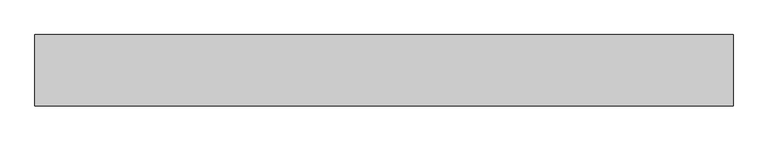
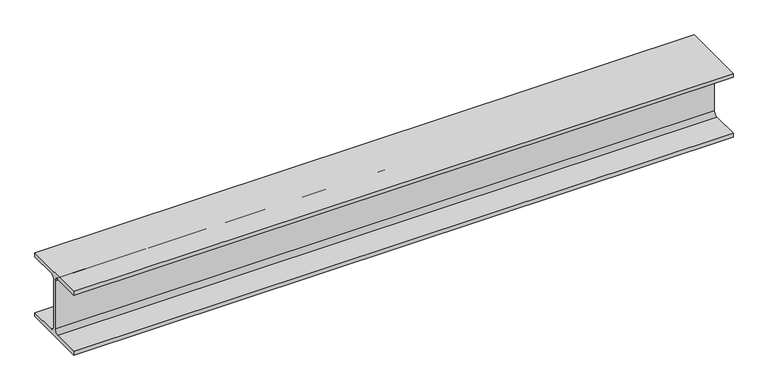
"""IFC4 building model written with IfcOpenShell, lengths in millimetres: beam geometry, 0912_Steel Framing_H-KSD3502 : H_SB_ASB_H-200x200x8x12."""

from ifc_helpers import new_model, si_unit, point, frame, frame_2d, origin, place, context, project, spatial, polyline, circle_curve, trimmed, segment, composite_curve, outline, extrude, source, transform, mapped, element, save


def beam_1032c180(model_context):
    return source(origin(), model_context, "Body", "SweptSolid", [
        extrude(outline(composite_curve([segment(polyline([(100.0, -88.0), (100.0, -100.0), (-100.0, -100.0), (-100.0, -88.0), (-17.0, -88.0)]), True, "CONTINUOUS"), segment(trimmed(circle_curve(frame_2d((-17.0, -75.0)), 13.0), [point((-17.0, -88.0))], [point((-4.0, -75.0))], True, "CARTESIAN"), True, "CONTINUOUS"), segment(polyline([(-4.0, -75.0), (-4.0, 75.0)]), True, "CONTINUOUS"), segment(trimmed(circle_curve(frame_2d((-17.0, 75.0)), 13.0), [point((-4.0, 75.0))], [point((-17.0, 88.0))], True, "CARTESIAN"), True, "CONTINUOUS"), segment(polyline([(-17.0, 88.0), (-100.0, 88.0), (-100.0, 100.0), (100.0, 100.0), (100.0, 88.0), (17.0, 88.0)]), True, "CONTINUOUS"), segment(trimmed(circle_curve(frame_2d((17.0, 75.0)), 13.0), [point((17.0, 88.0))], [point((4.0, 75.0))], True, "CARTESIAN"), True, "CONTINUOUS"), segment(polyline([(4.0, 75.0), (4.0, -75.0)]), True, "CONTINUOUS"), segment(trimmed(circle_curve(frame_2d((17.0, -75.0)), 13.0), [point((4.0, -75.0))], [point((17.0, -88.0))], True, "CARTESIAN"), True, "CONTINUOUS"), segment(polyline([(17.0, -88.0), (100.0, -88.0)]), True, "CONTINUOUS")], self_intersect=False)), frame((-926.5182437, 0.0, 0.0), z_axis=(1.0, 0.0, 0.0), x_axis=(0.0, 1.0, 0.0)), (0.0, 0.0, 1.0), 1959.1715213),
    ])


if __name__ == "__main__":
    model = new_model("IFC4")
    model_context = context("Model", 3, world=origin())
    ifc_project = project(units=[si_unit("LENGTHUNIT", "METRE", prefix="MILLI")], contexts=[model_context])
    site = spatial("IfcSite", under=ifc_project)
    building = spatial("IfcBuilding", under=site)
    placement = place(None, origin())
    beam_shape = beam_1032c180(model_context)
    element("IfcBeam", 1, ObjectType="0912_Steel Framing_H-KSD3502 : H_SB_ASB_H-200x200x8x12", at=placement, inside=building, context=model_context, shape_type="MappedRepresentation", body=[
        mapped(beam_shape, transform((0.0, 0.0, 0.0), x_axis=(1.0, 0.0, 0.0), y_axis=(0.0, 1.0, 0.0), z_axis=(0.0, 0.0, 1.0))),
    ])
    save(model, "model.ifc")

# Revit data of these elements
# Type "0912_Steel Framing_H-KSD3502 : H_SB_ASB_H-200x200x8x12"
#   H_WM Code_1 = "S01AA002-00001 | Main Steel Structure Fabrication Work | Shelter/Building | Medium Steel - Standard (90KG/M>Weight≥30KG/M) | Material: (   )"
#   H_WM Code_2 = "S03AA028-00001 | Main Steel Structure Erection Work | Shelter/Building | Medium Steel (90KG/M>Weight≥30KG/M) | Material: (   )"
#   H_WM Code_3 = "S01AA010-00001 | Main Steel Structure Fabrication Work | Shelter/Building | Steel Painting/Coating | for Non-Fireproofed Steel Surface, Surface Preparation, Primer, Second & Final Coat | Material: (   )"
#   H_Q'ty Cal Type Tag = "SB-Q2"
#   Width = 20.0 cm
#   Web Thickness = 0.8 cm
#   Web Fillet = 1.3 cm
#   Warping Constant = 141000.0 cm⁶
#   W = 0
#   Torsional Moment of Inertia = 26.2485 cm⁴
#   Section Area = 63.53 cm²
#   Plastic Modulus weak axis = 244.0 cm³
#   Plastic Modulus strong axis = 525.0 cm³
#   Perimeter = 1.16 m²/m
#   Nominal Weight = 49.90 kgf/m
#   Moment of Inertia weak axis = 1600.00 cm⁴
#   Moment of Inertia strong axis = 4720.00 cm⁴
#   Height = 20.0 cm
#   Flange Thickness = 1.2 cm
#   Elastic Modulus weak axis = 160.0 cm³
#   Elastic Modulus strong axis = 472.0 cm³
#   Centroid Vertical = 10.0 cm
#   Centroid Horizontal = 10.0 cm
#   Ix = 47200000
#   Length [instance default] = 1.5240 m
#   Zx = 525000
#   b = 0.2000 m
#   h = 0.2000 m
#   r = 0.0130 m
#   s = 0.0080 m
#   t = 0.0120 m
#   A = 0.006353 m²
#   Structural Material [instance default] = Steel, 45-345
#   Assembly Code = ""
# Element 1 (IfcBeam, "0912_Steel Framing_H-KSD3502 : H_SB_ASB_H-200x200x8x12")
#   Structural Material = none
# Materials
#   "Steel, 45-345": class "Metal", colour RGB 189 187 185, transparency 0, Description = "Steel 345 MPa", Cost = 0
